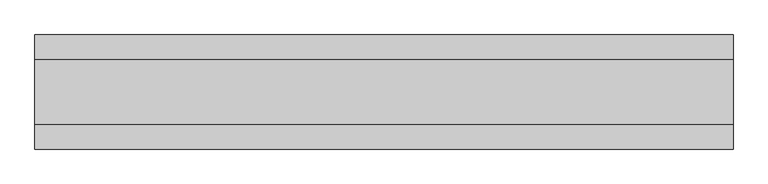
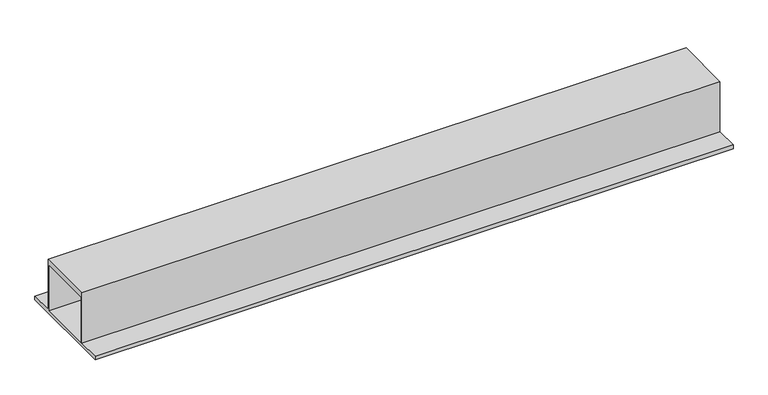
"""IFC4 building model written with IfcOpenShell, lengths in millimetres: beam geometry, NLRS_28_SF_LIB_stalen ligger THQ-AV-CWV-MMBS-SRP_gen_rsf : stalen ligger_gen__THQ_280x10-290x30-550x20."""

from ifc_helpers import new_model, si_unit, frame, origin, place, context, project, spatial, polyline, outline, extrude, source, transform, mapped, element, save


def beam_09e22bfa(model_context):
    return source(origin(), model_context, "Body", "SweptSolid", [
        extrude(outline(polyline([(143.5, 280.0), (143.5, 0.0), (263.5, 0.0), (263.5, -20.0), (-286.5, -20.0), (-286.5, 0.0), (-166.5, 0.0), (-166.5, 280.0), (143.5, 280.0)]), holes=[polyline([(133.5, 0.0), (133.5, 250.0), (-156.5, 250.0), (-156.5, 0.0), (133.5, 0.0)])]), frame((-1682.5, 0.0, 0.0), z_axis=(1.0, 0.0, 0.0), x_axis=(0.0, 1.0, 0.0)), (0.0, 0.0, 1.0), 3365.0),
    ])


if __name__ == "__main__":
    model = new_model("IFC4")
    model_context = context("Model", 3, world=origin())
    ifc_project = project(units=[si_unit("LENGTHUNIT", "METRE", prefix="MILLI")], contexts=[model_context])
    site = spatial("IfcSite", under=ifc_project)
    building = spatial("IfcBuilding", under=site)
    placement = place(None, origin())
    beam_shape = beam_09e22bfa(model_context)
    element("IfcBeam", 1, ObjectType="NLRS_28_SF_LIB_stalen ligger THQ-AV-CWV-MMBS-SRP_gen_rsf : stalen ligger_gen__THQ_280x10-290x30-550x20", at=placement, inside=building, context=model_context, shape_type="MappedRepresentation", body=[
        mapped(beam_shape, transform((0.0, 0.0, 0.0), x_axis=(1.0, 0.0, 0.0), y_axis=(0.0, 1.0, 0.0), z_axis=(0.0, 0.0, 1.0))),
    ])
    save(model, "model.ifc")

# Revit data of these elements
# Type "NLRS_28_SF_LIB_stalen ligger THQ-AV-CWV-MMBS-SRP_gen_rsf : stalen ligger_gen__THQ_280x10-290x30-550x20"
#   Export Type to IFC As = "IfcBeamType"
#   Type IfcGUID = "2GRbcre991teoKeCLB8MAm"
#   Type Comments = "THQ 280x10-290x30-550x20"
#   Model = " "
#   Manufacturer = " "
#   Fire Rating = " "
#   Description = "stalen ligger THQ 280x10-290x30-550x20"
#   Assembly Code = "28.11"
#   tw = 10 mm
#   tu = 20 mm
#   to = 30 mm
#   h = 280 mm
#   bu = 550 mm
#   bo = 290 mm
#   NLRS_C_lengte [instance default] = 1500 mm
#   Length [instance default] = 1500 mm
#   RSF_C_vullen_met_beton [instance default] = no
#   RSF_C_petligger = no
#   RSF_C_hoedligger = yes
#   Structural Material = NLRS_h2_staal_gen_rsf
#   Keynote = ""
# Element 1 (IfcBeam, "NLRS_28_SF_LIB_stalen ligger THQ-AV-CWV-MMBS-SRP_gen_rsf : stalen ligger_gen__THQ_280x10-290x30-550x20")
#   NLRS_C_lengte = 3365 mm
#   Materials on its faces: "NLRS_h2_staal_gen_rsf"
# Materials
#   "NLRS_h2_staal_gen_rsf": class "H - Metaal", colour RGB 189 187 185, transparency 0, Keynote = "h2", Manufacturer = "Revit Standards Foundation", URL = "www.revitstandards.org", Description = "staal", Cost = 0
